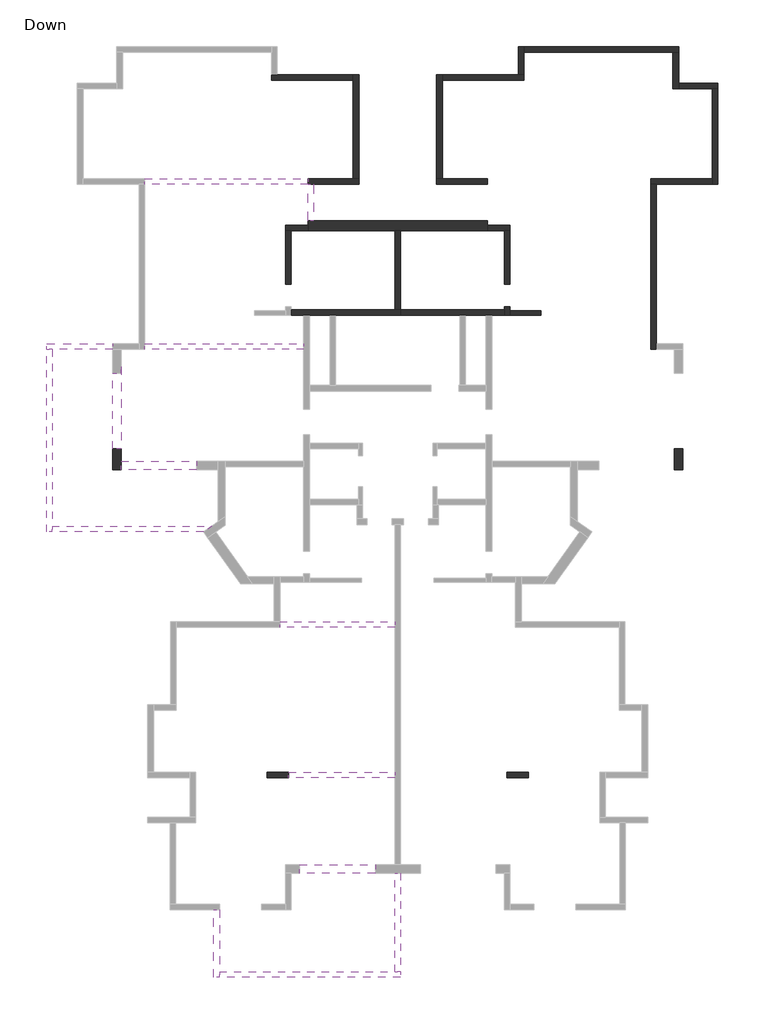
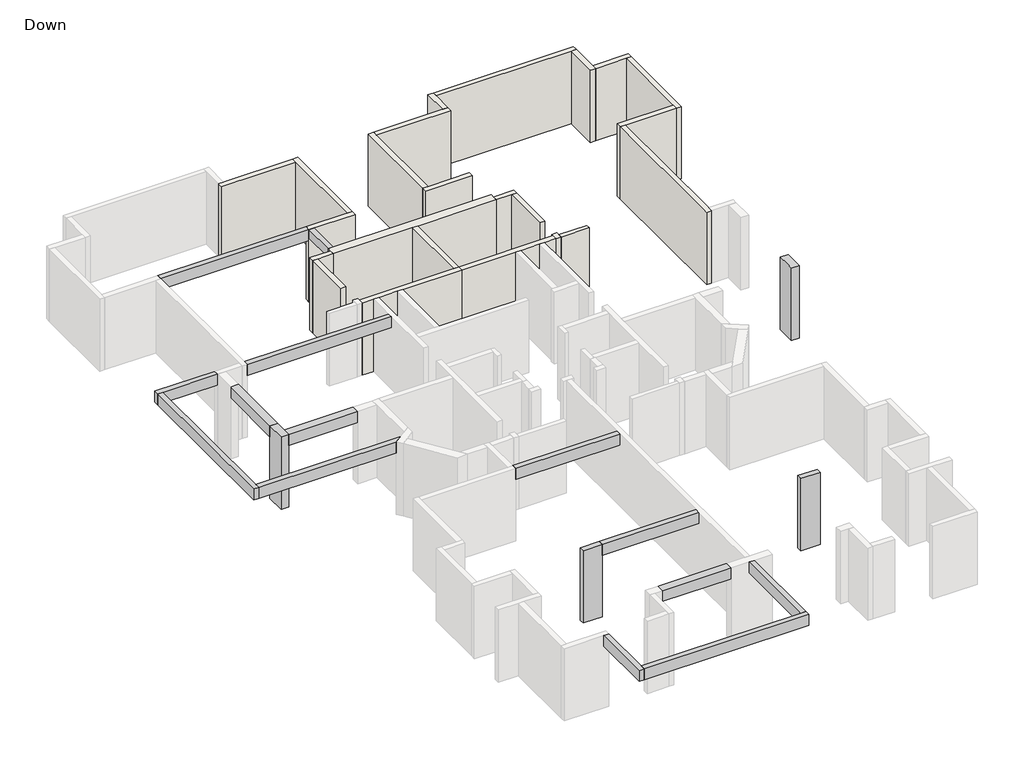
# One storey, part 3 of 3: 23 walls, 14 beams, 4 columns.
"""IFC4 building model written with IfcOpenShell, lengths in millimetres."""

from ifc_helpers import new_model, si_unit, origin, place, context, project, spatial, faceted_brep, element, save

model = new_model("IFC4")

# Units and contexts
model_context = context("Model", 3, world=origin())
ifc_project = project(units=[si_unit("LENGTHUNIT", "METRE", prefix="MILLI")], contexts=[model_context])

# Site, building, storey
site = spatial("IfcSite", under=ifc_project)
building = spatial("IfcBuilding", under=site)
storey = spatial("IfcBuildingStorey", under=building, Name="Down", Elevation=0.0)

# Beams
placement = place(None, origin())
element("IfcBeam", 1, ObjectType="Concrete Rectengular Beam : 20/35", at=placement, inside=storey, context=model_context, shape_type="Brep", body=[
    faceted_brep([(1026.9065089, 5707.9881624, 3000.0), (826.9065089, 5707.9881624, 3000.0), (826.9065089, 4410.637169, 3000.0), (1026.9065089, 4410.637169, 3000.0), (826.9065089, 5707.9881624, 2800.0), (826.9065089, 5707.9881624, 2650.0), (826.9065089, 4410.637169, 2650.0), (1026.9065089, 5707.9881624, 2650.0), (1026.9065089, 4410.637169, 2650.0)], [[[0, 1, 2, 3]], [[1, 4, 5, 6, 2]], [[5, 7, 8, 6]], [[7, 0, 3, 8]], [[1, 0, 7, 5, 4]], [[3, 2, 6, 8]]]),
])
element("IfcBeam", 2, ObjectType="Concrete Rectengular Beam : 20/45", at=placement, inside=storey, context=model_context, shape_type="Brep", body=[
    faceted_brep([(-4977.0670011, 46.6636591, 3000.0), (-4977.0670011, -153.3363409, 3000.0), (675.9131314, -153.3363409, 3000.0), (675.9131314, 46.6636591, 3000.0), (-4977.0670011, -153.3363409, 2550.0), (675.9131314, -153.3363409, 2550.0), (675.9131314, -153.3363409, 2800.0), (-4977.0670011, 46.6636591, 2550.0), (675.9131314, 46.6636591, 2550.0), (-4977.0670011, 46.6636591, 2800.0), (675.9131314, 46.6636591, 2800.0)], [[[0, 1, 2, 3]], [[1, 4, 5, 6, 2]], [[4, 7, 8, 5]], [[7, 9, 0, 3, 10, 8]], [[1, 0, 9, 7, 4]], [[3, 2, 6, 5, 8, 10]]]),
])
element("IfcBeam", 3, ObjectType="Concrete Rectengular Beam : 20/45", at=placement, inside=storey, context=model_context, shape_type="Brep", body=[
    faceted_brep([(-8477.9594861, 46.6636591, 3000.0), (-8477.9594861, -153.3363409, 3000.0), (-8277.9594861, -153.3363409, 3000.0), (-6127.9594861, -153.3363409, 3000.0), (-6127.9594861, 46.6636591, 3000.0), (-8477.9594861, 46.6636591, 2550.0), (-6127.9594861, 46.6636591, 2550.0), (-8477.9594861, -153.3363409, 2550.0), (-6127.9594861, -153.3363409, 2550.0), (-8277.9594861, -153.3363409, 2550.0), (-6127.9594861, -153.3363409, 2800.0)], [[[0, 1, 2, 3, 4]], [[5, 0, 4, 6]], [[7, 5, 6, 8, 9]], [[1, 7, 9, 8, 10, 3, 2]], [[4, 3, 10, 8, 6]], [[1, 0, 5, 7]]]),
])
element("IfcBeam", 4, ObjectType="Concrete Rectengular Beam : 20/45", at=placement, inside=storey, context=model_context, shape_type="Brep", body=[
    faceted_brep([(-8477.9594861, -6653.3363409, 3000.0), (-8277.9594861, -6653.3363409, 3000.0), (-8277.9594861, -6453.3363409, 3000.0), (-8277.9594861, -153.3363409, 3000.0), (-8477.9594861, -153.3363409, 3000.0), (-8477.9594861, -6653.3363409, 2550.0), (-8477.9594861, -153.3363409, 2550.0), (-8277.9594861, -6653.3363409, 2550.0), (-8277.9594861, -153.3363409, 2550.0), (-8277.9594861, -6453.3363409, 2550.0), (-8277.9594861, -153.3363409, 2800.0)], [[[0, 1, 2, 3, 4]], [[5, 0, 4, 6]], [[7, 5, 6, 8, 9]], [[1, 7, 9, 8, 10, 3, 2]], [[4, 3, 10, 8, 6]], [[1, 0, 5, 7]]]),
])
element("IfcBeam", 5, ObjectType="Concrete Rectengular Beam : 20/45", at=placement, inside=storey, context=model_context, shape_type="Brep", body=[
    faceted_brep([(-2884.5731861, -6652.8905163, 3000.0), (-2604.1186694, -6453.3363409, 3000.0), (-8277.9594861, -6453.3363409, 3000.0), (-8277.9594861, -6653.3363409, 3000.0), (-2884.256416, -6653.3363409, 3000.0), (-2884.256416, -6653.3363409, 2550.0), (-8277.9594861, -6653.3363409, 2550.0), (-2604.1186694, -6453.3363409, 2550.0), (-2884.5731861, -6652.8905163, 2550.0), (-8277.9594861, -6453.3363409, 2550.0), (-2604.1186694, -6453.3363409, 2800.0), (-8277.9594861, -6453.3363409, 2800.0)], [[[0, 1, 2, 3, 4]], [[5, 4, 3, 6]], [[7, 8, 5, 6, 9]], [[1, 10, 7, 9, 11, 2]], [[0, 8, 7, 10, 1]], [[8, 0, 4, 5]], [[3, 2, 11, 9, 6]]]),
])
element("IfcBeam", 6, ObjectType="Concrete Rectengular Beam : 20/45", at=placement, inside=storey, context=model_context, shape_type="Brep", body=[
    faceted_brep([(-2525.0802461, -22500.6211091, 3000.0), (-2325.0802461, -22500.6211091, 3000.0), (-2325.0802461, -22300.6211091, 3000.0), (-2325.0802461, -20100.6211091, 3000.0), (-2525.0802461, -20100.6211091, 3000.0), (-2525.0802461, -22500.6211091, 2550.0), (-2525.0802461, -20100.6211091, 2550.0), (-2325.0802461, -22500.6211091, 2550.0), (-2325.0802461, -20100.6211091, 2550.0), (-2325.0802461, -22300.6211091, 2550.0), (-2325.0802461, -20100.6211091, 2800.0)], [[[0, 1, 2, 3, 4]], [[5, 0, 4, 6]], [[7, 5, 6, 8, 9]], [[1, 7, 9, 8, 10, 3, 2]], [[4, 3, 10, 8, 6]], [[1, 0, 5, 7]]]),
])
element("IfcBeam", 7, ObjectType="Concrete Rectengular Beam : 20/45", at=placement, inside=storey, context=model_context, shape_type="Brep", body=[
    faceted_brep([(4123.5952506, -22500.6211091, 3000.0), (4123.5952506, -22300.6211091, 3000.0), (3923.5952506, -22300.6211091, 3000.0), (-2325.0802461, -22300.6211091, 3000.0), (-2325.0802461, -22500.6211091, 3000.0), (4123.5952506, -22500.6211091, 2550.0), (-2325.0802461, -22500.6211091, 2550.0), (4123.5952506, -22300.6211091, 2550.0), (-2325.0802461, -22300.6211091, 2550.0), (3923.5952506, -22300.6211091, 2550.0), (-2325.0802461, -22300.6211091, 2800.0)], [[[0, 1, 2, 3, 4]], [[5, 0, 4, 6]], [[7, 5, 6, 8, 9]], [[1, 7, 9, 8, 10, 3, 2]], [[4, 3, 10, 8, 6]], [[1, 0, 5, 7]]]),
])
element("IfcBeam", 8, ObjectType="Concrete Rectengular Beam : 20/45", at=placement, inside=storey, context=model_context, shape_type="Brep", body=[
    faceted_brep([(4123.5952506, -18796.3164734, 3000.0), (3923.5952506, -18796.3164734, 3000.0), (3923.5952506, -22300.6211091, 3000.0), (4123.5952506, -22300.6211091, 3000.0), (4123.5952506, -18796.3164734, 2550.0), (4123.5952506, -18796.3164734, 2800.0), (4123.5952506, -22300.6211091, 2800.0), (4123.5952506, -22300.6211091, 2550.0), (3923.5952506, -18796.3164734, 2550.0), (3923.5952506, -22300.6211091, 2550.0), (3923.5952506, -18796.3164734, 2800.0), (3923.5952506, -22300.6211091, 2800.0)], [[[0, 1, 2, 3]], [[4, 5, 0, 3, 6, 7]], [[8, 4, 7, 9]], [[1, 10, 8, 9, 11, 2]], [[1, 0, 5, 4, 8, 10]], [[3, 2, 11, 9, 7, 6]]]),
])
element("IfcBeam", 9, ObjectType="Concrete Rectengular Beam : 20/45", at=placement, inside=storey, context=model_context, shape_type="Brep", body=[
    faceted_brep([(129.5813071, -15199.2157792, 3000.0), (129.5813071, -15399.2157792, 3000.0), (3923.5952506, -15399.2157792, 3000.0), (3923.5952506, -15199.2157792, 3000.0), (129.5813071, -15399.2157792, 2800.0), (129.5813071, -15399.2157792, 2550.0), (3923.5952506, -15399.2157792, 2550.0), (3923.5952506, -15399.2157792, 2800.0), (129.5813071, -15199.2157792, 2550.0), (3923.5952506, -15199.2157792, 2550.0), (3923.5952506, -15199.2157792, 2800.0), (129.5813071, -15199.2157792, 2800.0)], [[[0, 1, 2, 3]], [[2, 1, 4, 5, 6, 7]], [[5, 8, 9, 6]], [[0, 3, 10, 9, 8, 11]], [[1, 0, 11, 8, 5, 4]], [[3, 2, 7, 6, 9, 10]]]),
])
element("IfcBeam", 10, ObjectType="Concrete Rectengular Beam : 20/45", at=placement, inside=storey, context=model_context, shape_type="Brep", body=[
    faceted_brep([(3923.5952506, -10045.6542217, 3000.0), (3923.5952506, -9845.6542217, 3000.0), (-173.424617, -9845.6542217, 3000.0), (-173.424617, -10045.6542217, 3000.0), (3923.5952506, -10045.6542217, 2550.0), (3923.5952506, -10045.6542217, 2800.0), (-173.424617, -10045.6542217, 2550.0), (3923.5952506, -9845.6542217, 2550.0), (-173.424617, -9845.6542217, 2550.0), (3923.5952506, -9845.6542217, 2800.0), (-173.424617, -9845.6542217, 2800.0)], [[[0, 1, 2, 3]], [[4, 5, 0, 3, 6]], [[7, 4, 6, 8]], [[1, 9, 7, 8, 10, 2]], [[1, 0, 5, 4, 7, 9]], [[3, 2, 10, 8, 6]]]),
])
element("IfcBeam", 11, ObjectType="Concrete Rectengular Beam : 20/45", at=placement, inside=storey, context=model_context, shape_type="Brep", body=[
    faceted_brep([(826.9065089, 5707.9881624, 3000.0), (826.9065089, 5907.9881624, 3000.0), (-4977.0670011, 5907.9881624, 3000.0), (-4977.0670011, 5707.9881624, 3000.0), (826.9065089, 5707.9881624, 2550.0), (826.9065089, 5707.9881624, 2800.0), (-4977.0670011, 5707.9881624, 2800.0), (-4977.0670011, 5707.9881624, 2550.0), (826.9065089, 5907.9881624, 2550.0), (-4977.0670011, 5907.9881624, 2550.0)], [[[0, 1, 2, 3]], [[4, 5, 0, 3, 6, 7]], [[8, 4, 7, 9]], [[1, 8, 9, 2]], [[1, 0, 5, 4, 8]], [[3, 2, 9, 7, 6]]]),
])
element("IfcBeam", 12, ObjectType="Concrete Rectengular Beam : 30/45", at=placement, inside=storey, context=model_context, shape_type="Brep", body=[
    faceted_brep([(3223.9263764, -18796.3164734, 3000.0), (3223.9263764, -18796.3164734, 2550.0), (3223.9263764, -18496.3164734, 2550.0), (3223.9263764, -18496.3164734, 2800.0), (3223.9263764, -18496.3164734, 3000.0), (524.9197539, -18496.3164734, 3000.0), (524.9197539, -18796.3164734, 3000.0), (524.9197539, -18496.3164734, 2550.0), (524.9197539, -18496.3164734, 2800.0), (524.9197539, -18796.3164734, 2550.0)], [[[0, 1, 2, 3, 4]], [[0, 4, 5, 6]], [[5, 4, 3, 2, 7, 8]], [[2, 1, 9, 7]], [[1, 0, 6, 9]], [[6, 5, 8, 7, 9]]]),
])
element("IfcBeam", 13, ObjectType="Concrete Rectengular Beam : 30/45", at=placement, inside=storey, context=model_context, shape_type="Brep", body=[
    faceted_brep([(-5827.2121465, -4140.6873343, 3000.0), (-5827.2121465, -4440.6873343, 3000.0), (-3130.7912039, -4440.6873343, 3000.0), (-3130.7912039, -4140.6873343, 3000.0), (-5827.2121465, -4140.6873343, 2550.0), (-5827.2121465, -4140.6873343, 2800.0), (-3130.7912039, -4140.6873343, 2550.0), (-5827.2121465, -4440.6873343, 2550.0), (-3130.7912039, -4440.6873343, 2550.0), (-5827.2121465, -4440.6873343, 2800.0), (-3130.7912039, -4440.6873343, 2800.0)], [[[0, 1, 2, 3]], [[4, 5, 0, 3, 6]], [[7, 4, 6, 8]], [[2, 1, 9, 7, 8, 10]], [[1, 0, 5, 4, 7, 9]], [[3, 2, 10, 8, 6]]]),
])
element("IfcBeam", 14, ObjectType="Concrete Rectengular Beam : 30/45", at=placement, inside=storey, context=model_context, shape_type="Brep", body=[
    faceted_brep([(-5827.2121465, -770.4005958, 2550.0), (-5827.9594861, -770.4005958, 2550.0), (-5827.9594861, -770.4005958, 2800.0), (-5827.2121465, -770.4005958, 2800.0), (-6127.2121465, -1013.3363409, 3000.0), (-6127.2121465, -3690.6873343, 3000.0), (-5827.9594861, -3690.6873343, 3000.0), (-5827.9594861, -1013.3363409, 3000.0), (-5827.2121465, -3690.6873343, 2550.0), (-5827.2121465, -3690.6873343, 2800.0), (-6127.2121465, -3690.6873343, 2550.0), (-6127.2121465, -1013.3363409, 2550.0), (-5827.9594861, -1013.3363409, 2550.0), (-6127.2121465, -1013.3363409, 2800.0), (-6127.2121465, -3690.6873343, 2800.0), (-5827.9594861, -3690.6873343, 2800.0), (-5827.9594861, -1013.3363409, 2800.0)], [[[0, 1, 2, 3]], [[4, 5, 6, 7]], [[8, 0, 3, 9]], [[0, 8, 10, 11, 12, 1]], [[5, 4, 13, 11, 10, 14]], [[10, 8, 9, 15, 6, 5, 14]], [[1, 12, 16, 2]], [[4, 7, 16, 12, 11, 13]], [[16, 15, 9, 3, 2]], [[15, 16, 7, 6]]]),
])

# Columns
element("IfcColumn", 15, ObjectType="Concrete Rectengular Column : 20/75", at=placement, inside=storey, context=model_context, shape_type="Brep", body=[
    faceted_brep([(-620.4186929, -15199.2157792, 0.0), (129.5813071, -15199.2157792, 0.0), (129.5813071, -15399.2157792, 0.0), (-620.4186929, -15399.2157792, 0.0), (-620.4186929, -15199.2157792, 3000.0), (129.5813071, -15199.2157792, 3000.0), (-620.4186929, -15199.2157792, 2800.0), (129.5813071, -15399.2157792, 3000.0), (-620.4186929, -15399.2157792, 3000.0), (-620.4186929, -15399.2157792, 2800.0)], [[[0, 1, 2, 3]], [[4, 5, 1, 0, 6]], [[5, 7, 2, 1]], [[7, 8, 9, 3, 2]], [[8, 4, 6, 0, 3, 9]], [[4, 8, 7, 5]]]),
])
element("IfcColumn", 16, ObjectType="Concrete Rectengular Column : 20/75", at=placement, inside=storey, context=model_context, shape_type="Brep", body=[
    faceted_brep([(8667.6091941, -15199.2157792, 0.0), (8667.6091941, -15399.2157792, 0.0), (7917.6091941, -15399.2157792, 0.0), (7917.6091941, -15199.2157792, 0.0), (8667.6091941, -15199.2157792, 3000.0), (8667.6091941, -15199.2157792, 2800.0), (7917.6091941, -15199.2157792, 3000.0), (7917.6091941, -15399.2157792, 3000.0), (8667.6091941, -15399.2157792, 2800.0), (8667.6091941, -15399.2157792, 3000.0)], [[[0, 1, 2, 3]], [[4, 5, 0, 3, 6]], [[6, 3, 2, 7]], [[7, 2, 1, 8, 9]], [[9, 8, 1, 0, 5, 4]], [[4, 6, 7, 9]]]),
])
element("IfcColumn", 17, ObjectType="Concrete Rectengular Column : 30/75", at=placement, inside=storey, context=model_context, shape_type="Brep", body=[
    faceted_brep([(-5827.2121465, -3690.6873343, 0.0), (-5827.2121465, -4440.6873343, 0.0), (-6127.2121465, -4440.6873343, 0.0), (-6127.2121465, -3690.6873343, 0.0), (-5827.2121465, -3690.6873343, 3000.0), (-5827.2121465, -4140.6873343, 3000.0), (-5827.2121465, -4440.6873343, 3000.0), (-5827.2121465, -3690.6873343, 2800.0), (-6127.2121465, -4440.6873343, 3000.0), (-6127.2121465, -4440.6873343, 2800.0), (-6127.2121465, -3690.6873343, 3000.0), (-5827.9594861, -3690.6873343, 3000.0)], [[[0, 1, 2, 3]], [[4, 5, 6, 1, 0, 7]], [[6, 8, 9, 2, 1]], [[8, 10, 3, 2, 9]], [[10, 11, 4, 7, 0, 3]], [[4, 11, 10, 8, 6, 5]]]),
])
element("IfcColumn", 18, ObjectType="Concrete Rectengular Column : 30/75", at=placement, inside=storey, context=model_context, shape_type="Brep", body=[
    faceted_brep([(13874.4026477, -3690.6873343, 0.0), (14174.4026477, -3690.6873343, 0.0), (14174.4026477, -4440.6873343, 0.0), (13874.4026477, -4440.6873343, 0.0), (13874.4026477, -3690.6873343, 3000.0), (13874.4026477, -3690.6873343, 2800.0), (13874.4026477, -4440.6873343, 3000.0), (13874.4026477, -4140.6873343, 3000.0), (14174.4026477, -4440.6873343, 2800.0), (14174.4026477, -4440.6873343, 3000.0), (14174.4026477, -3690.6873343, 3000.0), (13875.1499872, -3690.6873343, 3000.0)], [[[0, 1, 2, 3]], [[4, 5, 0, 3, 6, 7]], [[6, 3, 2, 8, 9]], [[9, 8, 2, 1, 10]], [[10, 1, 0, 5, 4, 11]], [[4, 7, 6, 9, 10, 11]]]),
])

# Walls
element("IfcWall", 19, ObjectType="15", at=placement, inside=storey, context=model_context, shape_type="Brep", body=[
    faceted_brep([(8019.2906148, 1057.3259107, 0.0), (9120.2839923, 1057.3259107, 0.0), (9120.2839923, 1057.3259107, 2800.0), (9120.2839923, 1057.3259107, 3000.0), (8019.2906148, 1057.3259107, 3000.0), (8019.2906148, 1207.3259107, 0.0), (8019.2906148, 1207.3259107, 2800.0), (8019.2906148, 1207.3259107, 3000.0), (9120.2839923, 1207.3259107, 3000.0), (9120.2839923, 1207.3259107, 2800.0), (9120.2839923, 1207.3259107, 0.0)], [[[0, 1, 2, 3, 4]], [[5, 6, 7, 8, 9, 10]], [[1, 0, 5, 10]], [[3, 2, 1, 10, 9, 8]], [[4, 3, 8, 7]], [[0, 4, 7, 6, 5]]]),
])
element("IfcWall", 20, ObjectType="20", at=placement, inside=storey, context=model_context, shape_type="Brep", body=[
    faceted_brep([(826.9065089, 5707.9881624, 0.0), (2639.2609277, 5707.9881624, 0.0), (2639.2609277, 5707.9881624, 3000.0), (826.9065089, 5707.9881624, 3000.0), (826.9065089, 5707.9881624, 2550.0), (826.9065089, 5907.9881624, 0.0), (826.9065089, 5907.9881624, 2550.0), (826.9065089, 5907.9881624, 3000.0), (2439.2609277, 5907.9881624, 3000.0), (2639.2609277, 5907.9881624, 3000.0), (2639.2609277, 5907.9881624, 0.0), (2439.2609277, 5907.9881624, 0.0)], [[[0, 1, 2, 3, 4]], [[5, 6, 7, 8, 9, 10, 11]], [[1, 0, 5, 11, 10]], [[3, 2, 9, 8, 7]], [[0, 4, 3, 7, 6, 5]], [[2, 1, 10, 9]]]),
])
element("IfcWall", 21, ObjectType="20", at=placement, inside=storey, context=model_context, shape_type="Brep", body=[
    faceted_brep([(2639.2609277, 5907.9881624, 0.0), (2639.2609277, 9607.9881624, 0.0), (2639.2609277, 9607.9881624, 3000.0), (2639.2609277, 5907.9881624, 3000.0), (2439.2609277, 5907.9881624, 0.0), (2439.2609277, 5907.9881624, 2800.0), (2439.2609277, 5907.9881624, 3000.0), (2439.2609277, 9407.9881624, 3000.0), (2439.2609277, 9607.9881624, 3000.0), (2439.2609277, 9607.9881624, 0.0), (2439.2609277, 9407.9881624, 0.0)], [[[0, 1, 2, 3]], [[4, 5, 6, 7, 8, 9, 10]], [[1, 0, 4, 10, 9]], [[3, 2, 8, 7, 6]], [[0, 3, 6, 5, 4]], [[2, 1, 9, 8]]]),
])
element("IfcWall", 22, ObjectType="20", at=placement, inside=storey, context=model_context, shape_type="Brep", body=[
    faceted_brep([(2439.2609277, 9607.9881624, 0.0), (-275.4113719, 9607.9881624, 0.0), (-475.4113719, 9607.9881624, 0.0), (-475.4113719, 9607.9881624, 3000.0), (-275.4113719, 9607.9881624, 3000.0), (2439.2609277, 9607.9881624, 3000.0), (2439.2609277, 9407.9881624, 0.0), (2439.2609277, 9407.9881624, 2800.0), (2439.2609277, 9407.9881624, 3000.0), (-475.4113719, 9407.9881624, 3000.0), (-475.4113719, 9407.9881624, 2800.0), (-475.4113719, 9407.9881624, 0.0)], [[[0, 1, 2, 3, 4, 5]], [[6, 7, 8, 9, 10, 11]], [[2, 1, 0, 6, 11]], [[5, 4, 3, 9, 8]], [[0, 5, 8, 7, 6]], [[3, 2, 11, 10, 9]]]),
])
element("IfcWall", 23, ObjectType="20", at=placement, inside=storey, context=model_context, shape_type="Brep", body=[
    faceted_brep([(826.9065089, 4260.637169, 0.0), (27.8998864, 4260.637169, 0.0), (27.8998864, 4260.637169, 2800.0), (27.8998864, 4260.637169, 3000.0), (826.9065089, 4260.637169, 3000.0), (826.9065089, 4260.637169, 2800.0), (826.9065089, 4060.637169, 0.0), (826.9065089, 4060.637169, 3000.0), (227.8998864, 4060.637169, 3000.0), (27.8998864, 4060.637169, 3000.0), (27.8998864, 4060.637169, 0.0), (227.8998864, 4060.637169, 0.0)], [[[0, 1, 2, 3, 4, 5]], [[6, 7, 8, 9, 10, 11]], [[1, 0, 6, 11, 10]], [[4, 3, 9, 8, 7]], [[0, 5, 4, 7, 6]], [[3, 2, 1, 10, 9]]]),
])
element("IfcWall", 24, ObjectType="20", at=placement, inside=storey, context=model_context, shape_type="Brep", body=[
    faceted_brep([(27.8998864, 4060.637169, 0.0), (27.8998864, 2158.3192882, 0.0), (27.8998864, 2158.3192882, 2800.0), (27.8998864, 2158.3192882, 3000.0), (27.8998864, 4060.637169, 3000.0), (227.8998864, 4060.637169, 0.0), (227.8998864, 4060.637169, 2800.0), (227.8998864, 4060.637169, 3000.0), (227.8998864, 2158.3192882, 3000.0), (227.8998864, 2158.3192882, 2800.0), (227.8998864, 2158.3192882, 0.0)], [[[0, 1, 2, 3, 4]], [[5, 6, 7, 8, 9, 10]], [[1, 0, 5, 10]], [[3, 2, 1, 10, 9, 8]], [[4, 3, 8, 7]], [[0, 4, 7, 6, 5]]]),
])
element("IfcWall", 25, ObjectType="20", at=placement, inside=storey, context=model_context, shape_type="Brep", body=[
    faceted_brep([(227.8998864, 1057.3259107, 0.0), (675.9131314, 1057.3259107, 0.0), (875.9131314, 1057.3259107, 0.0), (1608.3634625, 1057.3259107, 0.0), (1808.3634625, 1057.3259107, 0.0), (4128.562138, 1057.3259107, 0.0), (4128.562138, 1057.3259107, 3000.0), (1808.3634625, 1057.3259107, 3000.0), (1608.3634625, 1057.3259107, 3000.0), (875.9131314, 1057.3259107, 3000.0), (675.9131314, 1057.3259107, 3000.0), (227.8998864, 1057.3259107, 3000.0), (227.8998864, 1257.3259107, 0.0), (227.8998864, 1257.3259107, 2800.0), (227.8998864, 1257.3259107, 3000.0), (3928.562138, 1257.3259107, 3000.0), (4128.562138, 1257.3259107, 3000.0), (4128.562138, 1257.3259107, 0.0), (3928.562138, 1257.3259107, 0.0)], [[[0, 1, 2, 3, 4, 5, 6, 7, 8, 9, 10, 11]], [[12, 13, 14, 15, 16, 17, 18]], [[5, 4, 3, 2, 1, 0, 12, 18, 17]], [[11, 10, 9, 8, 7, 6, 16, 15, 14]], [[0, 11, 14, 13, 12]], [[6, 5, 17, 16]]]),
])
element("IfcWall", 26, ObjectType="20", at=placement, inside=storey, context=model_context, shape_type="Brep", body=[
    faceted_brep([(4128.562138, 1257.3259107, 0.0), (4128.562138, 4060.637169, 0.0), (4128.562138, 4060.637169, 2800.0), (4128.562138, 4060.637169, 3000.0), (4128.562138, 1257.3259107, 3000.0), (4128.562138, 1257.3259107, 2800.0), (3928.562138, 1257.3259107, 0.0), (3928.562138, 1257.3259107, 2800.0), (3928.562138, 1257.3259107, 3000.0), (3928.562138, 4060.637169, 3000.0), (3928.562138, 4060.637169, 2800.0), (3928.562138, 4060.637169, 0.0)], [[[0, 1, 2, 3, 4, 5]], [[6, 7, 8, 9, 10, 11]], [[1, 0, 6, 11]], [[4, 3, 9, 8]], [[0, 5, 4, 8, 7, 6]], [[3, 2, 1, 11, 10, 9]]]),
])
element("IfcWall", 27, ObjectType="20", at=placement, inside=storey, context=model_context, shape_type="Brep", body=[
    faceted_brep([(7220.2839923, 5907.9881624, 0.0), (5607.9295735, 5907.9881624, 0.0), (5407.9295735, 5907.9881624, 0.0), (5407.9295735, 5907.9881624, 3000.0), (5607.9295735, 5907.9881624, 3000.0), (7220.2839923, 5907.9881624, 3000.0), (7220.2839923, 5907.9881624, 2550.0), (7220.2839923, 5707.9881624, 0.0), (7220.2839923, 5707.9881624, 2550.0), (7220.2839923, 5707.9881624, 3000.0), (5407.9295735, 5707.9881624, 3000.0), (5407.9295735, 5707.9881624, 0.0)], [[[0, 1, 2, 3, 4, 5, 6]], [[7, 8, 9, 10, 11]], [[2, 1, 0, 7, 11]], [[5, 4, 3, 10, 9]], [[0, 6, 5, 9, 8, 7]], [[3, 2, 11, 10]]]),
])
element("IfcWall", 28, ObjectType="20", at=placement, inside=storey, context=model_context, shape_type="Brep", body=[
    faceted_brep([(5607.9295735, 5907.9881624, 0.0), (5607.9295735, 9407.9881624, 0.0), (5607.9295735, 9607.9881624, 0.0), (5607.9295735, 9607.9881624, 3000.0), (5607.9295735, 9407.9881624, 3000.0), (5607.9295735, 5907.9881624, 3000.0), (5607.9295735, 5907.9881624, 2800.0), (5407.9295735, 5907.9881624, 0.0), (5407.9295735, 5907.9881624, 3000.0), (5407.9295735, 9607.9881624, 3000.0), (5407.9295735, 9607.9881624, 0.0)], [[[0, 1, 2, 3, 4, 5, 6]], [[7, 8, 9, 10]], [[2, 1, 0, 7, 10]], [[5, 4, 3, 9, 8]], [[0, 6, 5, 8, 7]], [[3, 2, 10, 9]]]),
])
element("IfcWall", 29, ObjectType="20", at=placement, inside=storey, context=model_context, shape_type="Brep", body=[
    faceted_brep([(5607.9295735, 9407.9881624, 0.0), (8522.6018731, 9407.9881624, 0.0), (8522.6018731, 9407.9881624, 2800.0), (8522.6018731, 9407.9881624, 3000.0), (5607.9295735, 9407.9881624, 3000.0), (5607.9295735, 9407.9881624, 2800.0), (5607.9295735, 9607.9881624, 0.0), (5607.9295735, 9607.9881624, 3000.0), (8322.6018731, 9607.9881624, 3000.0), (8522.6018731, 9607.9881624, 3000.0), (8522.6018731, 9607.9881624, 0.0), (8322.6018731, 9607.9881624, 0.0)], [[[0, 1, 2, 3, 4, 5]], [[6, 7, 8, 9, 10, 11]], [[1, 0, 6, 11, 10]], [[4, 3, 9, 8, 7]], [[0, 5, 4, 7, 6]], [[3, 2, 1, 10, 9]]]),
])
element("IfcWall", 30, ObjectType="20", at=placement, inside=storey, context=model_context, shape_type="Brep", body=[
    faceted_brep([(8522.6018731, 9607.9881624, 0.0), (8522.6018731, 10413.9484273, 0.0), (8522.6018731, 10613.9484273, 0.0), (8522.6018731, 10613.9484273, 3000.0), (8522.6018731, 10413.9484273, 3000.0), (8522.6018731, 9607.9881624, 3000.0), (8322.6018731, 9607.9881624, 0.0), (8322.6018731, 9607.9881624, 3000.0), (8322.6018731, 10613.9484273, 3000.0), (8322.6018731, 10613.9484273, 0.0)], [[[0, 1, 2, 3, 4, 5]], [[6, 7, 8, 9]], [[2, 1, 0, 6, 9]], [[5, 4, 3, 8, 7]], [[0, 5, 7, 6]], [[3, 2, 9, 8]]]),
])
element("IfcWall", 31, ObjectType="20", at=placement, inside=storey, context=model_context, shape_type="Brep", body=[
    faceted_brep([(8522.6018731, 10413.9484273, 0.0), (13822.6018731, 10413.9484273, 0.0), (14022.6018731, 10413.9484273, 0.0), (14022.6018731, 10413.9484273, 3000.0), (13822.6018731, 10413.9484273, 3000.0), (8522.6018731, 10413.9484273, 3000.0), (8522.6018731, 10413.9484273, 2800.0), (8522.6018731, 10613.9484273, 0.0), (8522.6018731, 10613.9484273, 3000.0), (14022.6018731, 10613.9484273, 3000.0), (14022.6018731, 10613.9484273, 0.0)], [[[0, 1, 2, 3, 4, 5, 6]], [[7, 8, 9, 10]], [[2, 1, 0, 7, 10]], [[5, 4, 3, 9, 8]], [[0, 6, 5, 8, 7]], [[3, 2, 10, 9]]]),
])
element("IfcWall", 32, ObjectType="20", at=placement, inside=storey, context=model_context, shape_type="Brep", body=[
    faceted_brep([(13822.6018731, 10413.9484273, 0.0), (13822.6018731, 9110.3060432, 0.0), (13822.6018731, 9110.3060432, 2800.0), (13822.6018731, 9110.3060432, 3000.0), (13822.6018731, 10413.9484273, 3000.0), (13822.6018731, 10413.9484273, 2800.0), (14022.6018731, 10413.9484273, 0.0), (14022.6018731, 10413.9484273, 3000.0), (14022.6018731, 9310.3060432, 3000.0), (14022.6018731, 9110.3060432, 3000.0), (14022.6018731, 9110.3060432, 0.0), (14022.6018731, 9310.3060432, 0.0)], [[[0, 1, 2, 3, 4, 5]], [[6, 7, 8, 9, 10, 11]], [[1, 0, 6, 11, 10]], [[4, 3, 9, 8, 7]], [[0, 5, 4, 7, 6]], [[3, 2, 1, 10, 9]]]),
])
element("IfcWall", 33, ObjectType="20", at=placement, inside=storey, context=model_context, shape_type="Brep", body=[
    faceted_brep([(14022.6018731, 9110.3060432, 0.0), (15224.2575022, 9110.3060432, 0.0), (15424.2575022, 9110.3060432, 0.0), (15424.2575022, 9110.3060432, 3000.0), (15224.2575022, 9110.3060432, 3000.0), (14022.6018731, 9110.3060432, 3000.0), (14022.6018731, 9310.3060432, 0.0), (14022.6018731, 9310.3060432, 3000.0), (15424.2575022, 9310.3060432, 3000.0), (15424.2575022, 9310.3060432, 0.0)], [[[0, 1, 2, 3, 4, 5]], [[6, 7, 8, 9]], [[2, 1, 0, 6, 9]], [[5, 4, 3, 8, 7]], [[0, 5, 7, 6]], [[3, 2, 9, 8]]]),
])
element("IfcWall", 34, ObjectType="20", at=placement, inside=storey, context=model_context, shape_type="Brep", body=[
    faceted_brep([(15224.2575022, 9110.3060432, 0.0), (15224.2575022, 5907.9881624, 0.0), (15224.2575022, 5707.9881624, 0.0), (15224.2575022, 5707.9881624, 3000.0), (15224.2575022, 5907.9881624, 3000.0), (15224.2575022, 9110.3060432, 3000.0), (15224.2575022, 9110.3060432, 2800.0), (15424.2575022, 9110.3060432, 0.0), (15424.2575022, 9110.3060432, 3000.0), (15424.2575022, 5707.9881624, 3000.0), (15424.2575022, 5707.9881624, 0.0)], [[[0, 1, 2, 3, 4, 5, 6]], [[7, 8, 9, 10]], [[2, 1, 0, 7, 10]], [[5, 4, 3, 9, 8]], [[0, 6, 5, 8, 7]], [[3, 2, 10, 9]]]),
])
element("IfcWall", 35, ObjectType="20", at=placement, inside=storey, context=model_context, shape_type="Brep", body=[
    faceted_brep([(15224.2575022, 5907.9881624, 0.0), (13024.2575022, 5907.9881624, 0.0), (13024.2575022, 5907.9881624, 2550.0), (13024.2575022, 5907.9881624, 3000.0), (15224.2575022, 5907.9881624, 3000.0), (15224.2575022, 5907.9881624, 2800.0), (15224.2575022, 5707.9881624, 0.0), (15224.2575022, 5707.9881624, 3000.0), (13224.2575022, 5707.9881624, 3000.0), (13024.2575022, 5707.9881624, 3000.0), (13024.2575022, 5707.9881624, 2550.0), (13024.2575022, 5707.9881624, 0.0), (13224.2575022, 5707.9881624, 0.0)], [[[0, 1, 2, 3, 4, 5]], [[6, 7, 8, 9, 10, 11, 12]], [[1, 0, 6, 12, 11]], [[4, 3, 9, 8, 7]], [[0, 5, 4, 7, 6]], [[3, 2, 1, 11, 10, 9]]]),
])
element("IfcWall", 36, ObjectType="20", at=placement, inside=storey, context=model_context, shape_type="Brep", body=[
    faceted_brep([(13024.2575022, 5707.9881624, 0.0), (13024.2575022, -153.3363409, 0.0), (13024.2575022, -153.3363409, 3000.0), (13024.2575022, 46.6636591, 3000.0), (13024.2575022, 5707.9881624, 3000.0), (13024.2575022, 5707.9881624, 2800.0), (13224.2575022, 5707.9881624, 0.0), (13224.2575022, 5707.9881624, 3000.0), (13224.2575022, 46.6636591, 3000.0), (13224.2575022, -153.3363409, 3000.0), (13224.2575022, -153.3363409, 0.0), (13224.2575022, 46.6636591, 0.0)], [[[0, 1, 2, 3, 4, 5]], [[6, 7, 8, 9, 10, 11]], [[1, 0, 6, 11, 10]], [[4, 3, 2, 9, 8, 7]], [[0, 5, 4, 7, 6]], [[2, 1, 10, 9]]]),
])
element("IfcWall", 37, ObjectType="20", at=placement, inside=storey, context=model_context, shape_type="Brep", body=[
    faceted_brep([(7220.2839923, 4060.637169, 0.0), (7819.2906148, 4060.637169, 0.0), (8019.2906148, 4060.637169, 0.0), (8019.2906148, 4060.637169, 3000.0), (7819.2906148, 4060.637169, 3000.0), (7220.2839923, 4060.637169, 3000.0), (7220.2839923, 4260.637169, 0.0), (7220.2839923, 4260.637169, 2800.0), (7220.2839923, 4260.637169, 3000.0), (8019.2906148, 4260.637169, 3000.0), (8019.2906148, 4260.637169, 2800.0), (8019.2906148, 4260.637169, 0.0)], [[[0, 1, 2, 3, 4, 5]], [[6, 7, 8, 9, 10, 11]], [[2, 1, 0, 6, 11]], [[5, 4, 3, 9, 8]], [[0, 5, 8, 7, 6]], [[3, 2, 11, 10, 9]]]),
])
element("IfcWall", 38, ObjectType="20", at=placement, inside=storey, context=model_context, shape_type="Brep", body=[
    faceted_brep([(7819.2906148, 4060.637169, 0.0), (7819.2906148, 2158.3192882, 0.0), (7819.2906148, 2158.3192882, 2800.0), (7819.2906148, 2158.3192882, 3000.0), (7819.2906148, 4060.637169, 3000.0), (7819.2906148, 4060.637169, 2800.0), (8019.2906148, 4060.637169, 0.0), (8019.2906148, 4060.637169, 3000.0), (8019.2906148, 2158.3192882, 3000.0), (8019.2906148, 2158.3192882, 2800.0), (8019.2906148, 2158.3192882, 0.0)], [[[0, 1, 2, 3, 4, 5]], [[6, 7, 8, 9, 10]], [[1, 0, 6, 10]], [[3, 2, 1, 10, 9, 8]], [[4, 3, 8, 7]], [[0, 5, 4, 7, 6]]]),
])
element("IfcWall", 39, ObjectType="20", at=placement, inside=storey, context=model_context, shape_type="Brep", body=[
    faceted_brep([(7819.2906148, 1353.021275, 0.0), (7819.2906148, 1257.3259107, 0.0), (7819.2906148, 1057.3259107, 0.0), (7819.2906148, 1057.3259107, 3000.0), (7819.2906148, 1257.3259107, 3000.0), (7819.2906148, 1353.021275, 3000.0), (7819.2906148, 1353.021275, 2800.0), (8019.2906148, 1353.021275, 0.0), (8019.2906148, 1353.021275, 2800.0), (8019.2906148, 1353.021275, 3000.0), (8019.2906148, 1207.3259107, 3000.0), (8019.2906148, 1057.3259107, 3000.0), (8019.2906148, 1057.3259107, 0.0), (8019.2906148, 1207.3259107, 0.0)], [[[0, 1, 2, 3, 4, 5, 6]], [[7, 8, 9, 10, 11, 12, 13]], [[2, 1, 0, 7, 13, 12]], [[5, 4, 3, 11, 10, 9]], [[0, 6, 5, 9, 8, 7]], [[3, 2, 12, 11]]]),
])
element("IfcWall", 40, ObjectType="20", at=placement, inside=storey, context=model_context, shape_type="Brep", body=[
    faceted_brep([(7819.2906148, 1257.3259107, 0.0), (4128.562138, 1257.3259107, 0.0), (4128.562138, 1257.3259107, 2800.0), (4128.562138, 1257.3259107, 3000.0), (7819.2906148, 1257.3259107, 3000.0), (7819.2906148, 1257.3259107, 2800.0), (7819.2906148, 1057.3259107, 0.0), (7819.2906148, 1057.3259107, 3000.0), (7369.9528665, 1057.3259107, 3000.0), (7169.9528665, 1057.3259107, 3000.0), (6438.8270387, 1057.3259107, 3000.0), (6238.8270387, 1057.3259107, 3000.0), (4128.562138, 1057.3259107, 3000.0), (4128.562138, 1057.3259107, 0.0), (6238.8270387, 1057.3259107, 0.0), (6438.8270387, 1057.3259107, 0.0), (7169.9528665, 1057.3259107, 0.0), (7369.9528665, 1057.3259107, 0.0)], [[[0, 1, 2, 3, 4, 5]], [[6, 7, 8, 9, 10, 11, 12, 13, 14, 15, 16, 17]], [[1, 0, 6, 17, 16, 15, 14, 13]], [[4, 3, 12, 11, 10, 9, 8, 7]], [[0, 5, 4, 7, 6]], [[3, 2, 1, 13, 12]]]),
])
element("IfcWall", 41, ObjectType="35", at=placement, inside=storey, context=model_context, shape_type="Brep", body=[
    faceted_brep([(7220.2839923, 4410.637169, 0.0), (826.9065089, 4410.637169, 0.0), (826.9065089, 4410.637169, 3000.0), (7220.2839923, 4410.637169, 3000.0), (7220.2839923, 4060.637169, 0.0), (7220.2839923, 4060.637169, 3000.0), (4128.562138, 4060.637169, 3000.0), (3928.562138, 4060.637169, 3000.0), (826.9065089, 4060.637169, 3000.0), (826.9065089, 4060.637169, 0.0), (3928.562138, 4060.637169, 0.0), (4128.562138, 4060.637169, 0.0), (7220.2839923, 4260.637169, 0.0), (826.9065089, 4260.637169, 0.0), (826.9065089, 4260.637169, 3000.0), (7220.2839923, 4260.637169, 3000.0)], [[[0, 1, 2, 3]], [[4, 5, 6, 7, 8, 9, 10, 11]], [[1, 0, 12, 4, 11, 10, 9, 13]], [[2, 1, 13, 9, 8, 14]], [[3, 2, 14, 8, 7, 6, 5, 15]], [[0, 3, 15, 5, 4, 12]]]),
])

save(model, "model.ifc")

# Revit data of these elements
# Type "Concrete Rectengular Beam : 20/35"
#   Length [instance default] = 152.4 cm
#   b = 20 cm
#   h = 35 cm
#   Structural Material [instance default] = Concrete
#   Assembly Code = ""
# Type "Concrete Rectengular Beam : 20/45"
#   Length [instance default] = 152.4 cm
#   b = 20 cm
#   h = 45 cm
#   Structural Material [instance default] = Concrete
#   Assembly Code = ""
# Type "Concrete Rectengular Beam : 30/45"
#   Length [instance default] = 152.4 cm
#   b = 30 cm
#   h = 45 cm
#   Structural Material [instance default] = Concrete
#   Assembly Code = ""
# Type "Concrete Rectengular Column : 20/75"
#   b = 20 cm
#   h = 75 cm
#   Structural Material [instance default] = Concrete
# Type "Concrete Rectengular Column : 30/75"
#   b = 30 cm
#   h = 75 cm
#   Structural Material [instance default] = Concrete
# Type "15"
#   Layers, outside or top first: 15 cm "Concrete" (function 1)
# Type "20"
#   Layers, outside or top first: 20 cm "Concrete" (function 1)
# Type "35"
#   Layers, outside or top first: 35 cm "Concrete" (function 1)
# Element 1 (IfcBeam, "Concrete Rectengular Beam : 20/35")
#   Comments = ""
#   Mark = "B1"
#   SOFiSTiK_AMG_Comments = ""
#   SOFiSTiK_AMG_Scheduled = yes
#   SOFiSTiK_AMG_Adjusted = yes
#   Structural Material = Concrete
#   Phase Created = New Construction
#   Materials on its faces: "Concrete"
# Element 2 (IfcBeam, "Concrete Rectengular Beam : 20/45")
#   Comments = ""
#   Mark = "B3"
#   SOFiSTiK_AMG_Comments = ""
#   SOFiSTiK_AMG_Scheduled = yes
#   SOFiSTiK_AMG_Adjusted = yes
#   Structural Material = Concrete
#   Phase Created = New Construction
#   Materials on its faces: "Concrete"
# Element 3 (IfcBeam, "Concrete Rectengular Beam : 20/45")
#   Comments = ""
#   Mark = "B4"
#   SOFiSTiK_AMG_Comments = ""
#   SOFiSTiK_AMG_Scheduled = yes
#   SOFiSTiK_AMG_Adjusted = yes
#   Structural Material = Concrete
#   Phase Created = New Construction
#   Materials on its faces: "Concrete"
# Element 4 (IfcBeam, "Concrete Rectengular Beam : 20/45")
#   Comments = ""
#   Mark = "B5"
#   SOFiSTiK_AMG_Comments = ""
#   SOFiSTiK_AMG_Scheduled = yes
#   SOFiSTiK_AMG_Adjusted = yes
#   Structural Material = Concrete
#   Phase Created = New Construction
#   Materials on its faces: "Concrete"
# Element 5 (IfcBeam, "Concrete Rectengular Beam : 20/45")
#   Comments = ""
#   Mark = "B6"
#   SOFiSTiK_AMG_Comments = ""
#   SOFiSTiK_AMG_Scheduled = yes
#   SOFiSTiK_AMG_Adjusted = yes
#   Structural Material = Concrete
#   Phase Created = New Construction
#   Materials on its faces: "Concrete"
# Element 6 (IfcBeam, "Concrete Rectengular Beam : 20/45")
#   Comments = ""
#   Mark = "B7"
#   SOFiSTiK_AMG_Comments = ""
#   SOFiSTiK_AMG_Scheduled = yes
#   SOFiSTiK_AMG_Adjusted = yes
#   Structural Material = Concrete
#   Phase Created = New Construction
#   Materials on its faces: "Concrete"
# Element 7 (IfcBeam, "Concrete Rectengular Beam : 20/45")
#   Comments = ""
#   Mark = "B8"
#   SOFiSTiK_AMG_Comments = ""
#   SOFiSTiK_AMG_Scheduled = yes
#   SOFiSTiK_AMG_Adjusted = yes
#   Structural Material = Concrete
#   Phase Created = New Construction
#   Materials on its faces: "Concrete"
# Element 8 (IfcBeam, "Concrete Rectengular Beam : 20/45")
#   Comments = ""
#   Mark = "B9"
#   SOFiSTiK_AMG_Comments = ""
#   SOFiSTiK_AMG_Scheduled = yes
#   SOFiSTiK_AMG_Adjusted = yes
#   Structural Material = Concrete
#   Phase Created = New Construction
#   Materials on its faces: "Concrete"
# Element 9 (IfcBeam, "Concrete Rectengular Beam : 20/45")
#   Comments = ""
#   Mark = "B10"
#   SOFiSTiK_AMG_Comments = ""
#   SOFiSTiK_AMG_Scheduled = yes
#   SOFiSTiK_AMG_Adjusted = yes
#   Structural Material = Concrete
#   Phase Created = New Construction
#   Materials on its faces: "Concrete"
# Element 10 (IfcBeam, "Concrete Rectengular Beam : 20/45")
#   Comments = ""
#   Mark = "B11"
#   SOFiSTiK_AMG_Comments = ""
#   SOFiSTiK_AMG_Scheduled = yes
#   SOFiSTiK_AMG_Adjusted = yes
#   Structural Material = Concrete
#   Phase Created = New Construction
#   Materials on its faces: "Concrete"
# Element 11 (IfcBeam, "Concrete Rectengular Beam : 20/45")
#   Comments = ""
#   Mark = "B12"
#   SOFiSTiK_AMG_Comments = ""
#   SOFiSTiK_AMG_Scheduled = yes
#   SOFiSTiK_AMG_Adjusted = yes
#   Structural Material = Concrete
#   Phase Created = New Construction
#   Materials on its faces: "Concrete"
# Element 12 (IfcBeam, "Concrete Rectengular Beam : 30/45")
#   Comments = ""
#   Mark = "B23"
#   SOFiSTiK_AMG_Comments = ""
#   SOFiSTiK_AMG_Scheduled = yes
#   SOFiSTiK_AMG_Adjusted = yes
#   Structural Material = Concrete
#   Phase Created = New Construction
#   Materials on its faces: "Concrete"
# Element 13 (IfcBeam, "Concrete Rectengular Beam : 30/45")
#   Comments = ""
#   Mark = "B24"
#   SOFiSTiK_AMG_Comments = ""
#   SOFiSTiK_AMG_Scheduled = yes
#   SOFiSTiK_AMG_Adjusted = yes
#   Structural Material = Concrete
#   Phase Created = New Construction
#   Materials on its faces: "Concrete"
# Element 14 (IfcBeam, "Concrete Rectengular Beam : 30/45")
#   Comments = ""
#   Mark = "B25"
#   SOFiSTiK_AMG_Comments = ""
#   SOFiSTiK_AMG_Scheduled = yes
#   SOFiSTiK_AMG_Adjusted = yes
#   Structural Material = Concrete
#   Phase Created = New Construction
#   Materials on its faces: "Concrete"
# Element 15 (IfcColumn, "Concrete Rectengular Column : 20/75")
#   Comments = ""
#   Mark = "C3"
#   SOFiSTiK_AMG_Comments = ""
#   SOFiSTiK_AMG_Scheduled = yes
#   SOFiSTiK_AMG_Adjusted = yes
#   Structural Material = Concrete
#   Phase Created = New Construction
#   Materials on its faces: "Concrete"
# Element 16 (IfcColumn, "Concrete Rectengular Column : 20/75")
#   Comments = ""
#   Mark = "C4"
#   SOFiSTiK_AMG_Comments = ""
#   SOFiSTiK_AMG_Scheduled = yes
#   SOFiSTiK_AMG_Adjusted = yes
#   Structural Material = Concrete
#   Phase Created = New Construction
#   Materials on its faces: "Concrete"
# Element 17 (IfcColumn, "Concrete Rectengular Column : 30/75")
#   Comments = ""
#   Mark = "C5"
#   SOFiSTiK_AMG_Comments = ""
#   SOFiSTiK_AMG_Scheduled = yes
#   SOFiSTiK_AMG_Adjusted = yes
#   Structural Material = Concrete
#   Phase Created = New Construction
#   Materials on its faces: "Concrete"
# Element 18 (IfcColumn, "Concrete Rectengular Column : 30/75")
#   Comments = ""
#   Mark = "C6"
#   SOFiSTiK_AMG_Comments = ""
#   SOFiSTiK_AMG_Scheduled = yes
#   SOFiSTiK_AMG_Adjusted = yes
#   Structural Material = Concrete
#   Phase Created = New Construction
#   Materials on its faces: "Concrete"
# Element 19 (IfcWall, "15")
#   Comments = ""
#   Mark = "W94"
#   SOFiSTiK_AMG_Comments = ""
#   Top Offset = 0 cm
#   Base Offset = 0 cm
#   wall height = 300 cm
#   SOFiSTiK_AMG_Scheduled = yes
#   SOFiSTiK_AMG_Adjusted = yes
#   Phase Created = New Construction
#   Base Constraint = Down
#   Top Constraint = Typical Floor
#   Materials on its faces: "Concrete"
# Element 20 (IfcWall, "20")
#   Comments = ""
#   Mark = "W1"
#   SOFiSTiK_AMG_Comments = ""
#   Top Offset = 0 cm
#   Base Offset = 0 cm
#   wall height = 300 cm
#   SOFiSTiK_AMG_Scheduled = yes
#   SOFiSTiK_AMG_Adjusted = yes
#   Phase Created = New Construction
#   Base Constraint = Down
#   Top Constraint = Typical Floor
#   Materials on its faces: "Concrete"
# Element 21 (IfcWall, "20")
#   Comments = ""
#   Mark = "W2"
#   SOFiSTiK_AMG_Comments = ""
#   Top Offset = 0 cm
#   Base Offset = 0 cm
#   wall height = 300 cm
#   SOFiSTiK_AMG_Scheduled = yes
#   SOFiSTiK_AMG_Adjusted = yes
#   Phase Created = New Construction
#   Base Constraint = Down
#   Top Constraint = Typical Floor
#   Materials on its faces: "Concrete"
# Element 22 (IfcWall, "20")
#   Comments = ""
#   Mark = "W3"
#   SOFiSTiK_AMG_Comments = ""
#   Top Offset = 0 cm
#   Base Offset = 0 cm
#   wall height = 300 cm
#   SOFiSTiK_AMG_Scheduled = yes
#   SOFiSTiK_AMG_Adjusted = yes
#   Phase Created = New Construction
#   Base Constraint = Down
#   Top Constraint = Typical Floor
#   Materials on its faces: "Concrete"
# Element 23 (IfcWall, "20")
#   Comments = ""
#   Mark = "W12"
#   SOFiSTiK_AMG_Comments = ""
#   Top Offset = 0 cm
#   Base Offset = 0 cm
#   wall height = 300 cm
#   SOFiSTiK_AMG_Scheduled = yes
#   SOFiSTiK_AMG_Adjusted = yes
#   Phase Created = New Construction
#   Base Constraint = Down
#   Top Constraint = Typical Floor
#   Materials on its faces: "Concrete"
# Element 24 (IfcWall, "20")
#   Comments = ""
#   Mark = "W13"
#   SOFiSTiK_AMG_Comments = ""
#   Top Offset = 0 cm
#   Base Offset = 0 cm
#   wall height = 300 cm
#   SOFiSTiK_AMG_Scheduled = yes
#   SOFiSTiK_AMG_Adjusted = yes
#   Phase Created = New Construction
#   Base Constraint = Down
#   Top Constraint = Typical Floor
#   Materials on its faces: "Concrete"
# Element 25 (IfcWall, "20")
#   Comments = ""
#   Mark = "W15"
#   SOFiSTiK_AMG_Comments = ""
#   Top Offset = 0 cm
#   Base Offset = 0 cm
#   wall height = 300 cm
#   SOFiSTiK_AMG_Scheduled = yes
#   SOFiSTiK_AMG_Adjusted = yes
#   Phase Created = New Construction
#   Base Constraint = Down
#   Top Constraint = Typical Floor
#   Materials on its faces: "Concrete"
# Element 26 (IfcWall, "20")
#   Comments = ""
#   Mark = "W16"
#   SOFiSTiK_AMG_Comments = ""
#   Top Offset = 0 cm
#   Base Offset = 0 cm
#   wall height = 300 cm
#   SOFiSTiK_AMG_Scheduled = yes
#   SOFiSTiK_AMG_Adjusted = yes
#   Phase Created = New Construction
#   Base Constraint = Down
#   Top Constraint = Typical Floor
#   Materials on its faces: "Concrete"
# Element 27 (IfcWall, "20")
#   Comments = ""
#   Mark = "W42"
#   SOFiSTiK_AMG_Comments = ""
#   Top Offset = 0 cm
#   Base Offset = 0 cm
#   wall height = 300 cm
#   SOFiSTiK_AMG_Scheduled = yes
#   SOFiSTiK_AMG_Adjusted = yes
#   Phase Created = New Construction
#   Base Constraint = Down
#   Top Constraint = Typical Floor
#   Materials on its faces: "Concrete"
# Element 28 (IfcWall, "20")
#   Comments = ""
#   Mark = "W43"
#   SOFiSTiK_AMG_Comments = ""
#   Top Offset = 0 cm
#   Base Offset = 0 cm
#   wall height = 300 cm
#   SOFiSTiK_AMG_Scheduled = yes
#   SOFiSTiK_AMG_Adjusted = yes
#   Phase Created = New Construction
#   Base Constraint = Down
#   Top Constraint = Typical Floor
#   Materials on its faces: "Concrete"
# Element 29 (IfcWall, "20")
#   Comments = ""
#   Mark = "W44"
#   SOFiSTiK_AMG_Comments = ""
#   Top Offset = 0 cm
#   Base Offset = 0 cm
#   wall height = 300 cm
#   SOFiSTiK_AMG_Scheduled = yes
#   SOFiSTiK_AMG_Adjusted = yes
#   Phase Created = New Construction
#   Base Constraint = Down
#   Top Constraint = Typical Floor
#   Materials on its faces: "Concrete"
# Element 30 (IfcWall, "20")
#   Comments = ""
#   Mark = "W45"
#   SOFiSTiK_AMG_Comments = ""
#   Top Offset = 0 cm
#   Base Offset = 0 cm
#   wall height = 300 cm
#   SOFiSTiK_AMG_Scheduled = yes
#   SOFiSTiK_AMG_Adjusted = yes
#   Phase Created = New Construction
#   Base Constraint = Down
#   Top Constraint = Typical Floor
#   Materials on its faces: "Concrete"
# Element 31 (IfcWall, "20")
#   Comments = ""
#   Mark = "W46"
#   SOFiSTiK_AMG_Comments = ""
#   Top Offset = 0 cm
#   Base Offset = 0 cm
#   wall height = 300 cm
#   SOFiSTiK_AMG_Scheduled = yes
#   SOFiSTiK_AMG_Adjusted = yes
#   Phase Created = New Construction
#   Base Constraint = Down
#   Top Constraint = Typical Floor
#   Materials on its faces: "Concrete"
# Element 32 (IfcWall, "20")
#   Comments = ""
#   Mark = "W47"
#   SOFiSTiK_AMG_Comments = ""
#   Top Offset = 0 cm
#   Base Offset = 0 cm
#   wall height = 300 cm
#   SOFiSTiK_AMG_Scheduled = yes
#   SOFiSTiK_AMG_Adjusted = yes
#   Phase Created = New Construction
#   Base Constraint = Down
#   Top Constraint = Typical Floor
#   Materials on its faces: "Concrete"
# Element 33 (IfcWall, "20")
#   Comments = ""
#   Mark = "W48"
#   SOFiSTiK_AMG_Comments = ""
#   Top Offset = 0 cm
#   Base Offset = 0 cm
#   wall height = 300 cm
#   SOFiSTiK_AMG_Scheduled = yes
#   SOFiSTiK_AMG_Adjusted = yes
#   Phase Created = New Construction
#   Base Constraint = Down
#   Top Constraint = Typical Floor
#   Materials on its faces: "Concrete"
# Element 34 (IfcWall, "20")
#   Comments = ""
#   Mark = "W49"
#   SOFiSTiK_AMG_Comments = ""
#   Top Offset = 0 cm
#   Base Offset = 0 cm
#   wall height = 300 cm
#   SOFiSTiK_AMG_Scheduled = yes
#   SOFiSTiK_AMG_Adjusted = yes
#   Phase Created = New Construction
#   Base Constraint = Down
#   Top Constraint = Typical Floor
#   Materials on its faces: "Concrete"
# Element 35 (IfcWall, "20")
#   Comments = ""
#   Mark = "W50"
#   SOFiSTiK_AMG_Comments = ""
#   Top Offset = 0 cm
#   Base Offset = 0 cm
#   wall height = 300 cm
#   SOFiSTiK_AMG_Scheduled = yes
#   SOFiSTiK_AMG_Adjusted = yes
#   Phase Created = New Construction
#   Base Constraint = Down
#   Top Constraint = Typical Floor
#   Materials on its faces: "Concrete"
# Element 36 (IfcWall, "20")
#   Comments = ""
#   Mark = "W51"
#   SOFiSTiK_AMG_Comments = ""
#   Top Offset = 0 cm
#   Base Offset = 0 cm
#   wall height = 300 cm
#   SOFiSTiK_AMG_Scheduled = yes
#   SOFiSTiK_AMG_Adjusted = yes
#   Phase Created = New Construction
#   Base Constraint = Down
#   Top Constraint = Typical Floor
#   Materials on its faces: "Concrete"
# Element 37 (IfcWall, "20")
#   Comments = ""
#   Mark = "W53"
#   SOFiSTiK_AMG_Comments = ""
#   Top Offset = 0 cm
#   Base Offset = 0 cm
#   wall height = 300 cm
#   SOFiSTiK_AMG_Scheduled = yes
#   SOFiSTiK_AMG_Adjusted = yes
#   Phase Created = New Construction
#   Base Constraint = Down
#   Top Constraint = Typical Floor
#   Materials on its faces: "Concrete"
# Element 38 (IfcWall, "20")
#   Comments = ""
#   Mark = "W54"
#   SOFiSTiK_AMG_Comments = ""
#   Top Offset = 0 cm
#   Base Offset = 0 cm
#   wall height = 300 cm
#   SOFiSTiK_AMG_Scheduled = yes
#   SOFiSTiK_AMG_Adjusted = yes
#   Phase Created = New Construction
#   Base Constraint = Down
#   Top Constraint = Typical Floor
#   Materials on its faces: "Concrete"
# Element 39 (IfcWall, "20")
#   Comments = ""
#   Mark = "W55"
#   SOFiSTiK_AMG_Comments = ""
#   Top Offset = 0 cm
#   Base Offset = 0 cm
#   wall height = 300 cm
#   SOFiSTiK_AMG_Scheduled = yes
#   SOFiSTiK_AMG_Adjusted = yes
#   Phase Created = New Construction
#   Base Constraint = Down
#   Top Constraint = Typical Floor
#   Materials on its faces: "Concrete"
# Element 40 (IfcWall, "20")
#   Comments = ""
#   Mark = "W56"
#   SOFiSTiK_AMG_Comments = ""
#   Top Offset = 0 cm
#   Base Offset = 0 cm
#   wall height = 300 cm
#   SOFiSTiK_AMG_Scheduled = yes
#   SOFiSTiK_AMG_Adjusted = yes
#   Phase Created = New Construction
#   Base Constraint = Down
#   Top Constraint = Typical Floor
#   Materials on its faces: "Concrete"
# Element 41 (IfcWall, "35")
#   Comments = ""
#   Mark = "W87"
#   SOFiSTiK_AMG_Comments = ""
#   Top Offset = 0 cm
#   Base Offset = 0 cm
#   wall height = 300 cm
#   SOFiSTiK_AMG_Scheduled = yes
#   SOFiSTiK_AMG_Adjusted = yes
#   Phase Created = New Construction
#   Base Constraint = Down
#   Top Constraint = Typical Floor
#   Materials on its faces: "Concrete"
# Materials
#   "Concrete": class "Concrete", colour RGB 192 192 192, transparency 0, Keynote = "01000", Description = "Cast-in-place concrete", Cost = 0
